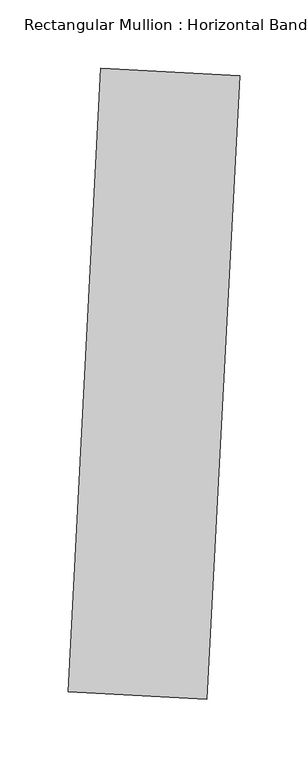
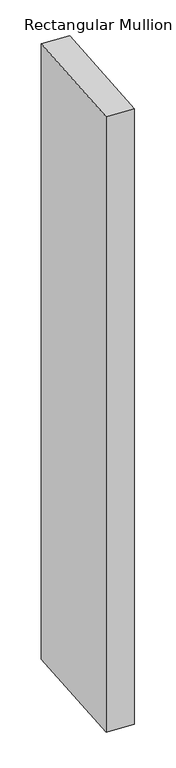
"""IFC4 building model written with IfcOpenShell, lengths in millimetres: member geometry, Rectangular Mullion : Horizontal Band."""

import ifcopenshell
import ifcopenshell.guid

model = None  # the IFC model being written
_history = None  # IfcOwnerHistory: only IFC2X3 demands one
_inside = {}  # id of a spatial element -> (the spatial element, [elements in it])
_under = {}  # id of a project, library or spatial element -> (it, [spatial elements below it])
_declared = {}  # id of a project -> (the project, [libraries it declares])
_typed = {}  # id of a type object -> (the type object, [elements of that type])
_made_of = {}  # id of a material, layer set ... -> (it, [elements and type objects made of it])


def new_model(schema):
    """Start an empty IFC model of exactly this schema.

    Asked for "IFC4X3", IfcOpenShell would pick the latest addendum, in which some entities
    have other attributes; the version numbers below select the first issue.
    IFC2X3 requires an IfcOwnerHistory on every rooted entity: one is made here for all.
    """
    global model, _history
    if schema == "IFC4X3":
        model = ifcopenshell.file(schema_version=(4, 3, 0, 0))
    else:
        model = ifcopenshell.file(schema=schema)
    _inside.clear()
    _under.clear()
    _declared.clear()
    _typed.clear()
    _made_of.clear()
    _history = None
    if model.schema == "IFC2X3":
        org = make("IfcOrganization", Name="unknown")
        user = make(
            "IfcPersonAndOrganization",
            ThePerson=make("IfcPerson", FamilyName="unknown"),
            TheOrganization=org,
        )
        app = make(
            "IfcApplication",
            ApplicationDeveloper=org,
            Version="unknown",
            ApplicationFullName="unknown",
            ApplicationIdentifier="unknown",
        )
        _history = make(
            "IfcOwnerHistory",
            OwningUser=user,
            OwningApplication=app,
            ChangeAction="ADDED",
            CreationDate=0,
        )
    return model


def make(cls, **values):
    """One entity of the class cls with the attributes given. An attribute that is None is left unset."""
    return model.create_entity(
        cls, **{name: value for name, value in values.items() if value is not None}
    )


def rooted(cls, **values):
    """An entity with a GlobalId (a new one), such as an element, a storey or a relation."""
    return make(cls, GlobalId=ifcopenshell.guid.new(), OwnerHistory=_history, **values)


def si_unit(unit_type, name, prefix=None):
    """IfcSIUnit, for example si_unit("LENGTHUNIT", "METRE", prefix="MILLI")."""
    return make("IfcSIUnit", UnitType=unit_type, Prefix=prefix, Name=name)


def assignment(units):
    """IfcUnitAssignment: the units of a project."""
    return None if units is None else make("IfcUnitAssignment", Units=units)


def point(xyz):
    """IfcCartesianPoint."""
    return None if xyz is None else make("IfcCartesianPoint", Coordinates=xyz)


def direction(xyz):
    """IfcDirection."""
    return None if xyz is None else make("IfcDirection", DirectionRatios=xyz)


def frame(location, z_axis=None, x_axis=None):
    """IfcAxis2Placement3D, a coordinate frame: its origin and axes. An axis left out is left unset."""
    return make(
        "IfcAxis2Placement3D",
        Location=point(location),
        Axis=direction(z_axis),
        RefDirection=direction(x_axis),
    )


def origin():
    """The frame at (0, 0, 0) with its axes left unset."""
    return frame((0.0, 0.0, 0.0))


def place(relative_to, where):
    """IfcLocalPlacement: puts the frame where relative to a parent placement (None: the world)."""
    return make(
        "IfcLocalPlacement", PlacementRelTo=relative_to, RelativePlacement=where
    )


def context(
    kind, dimensions, precision=None, world=None, true_north=None, identifier=None
):
    """IfcGeometricRepresentationContext, for example the 3D "Model" context."""
    return make(
        "IfcGeometricRepresentationContext",
        ContextIdentifier=identifier,
        ContextType=kind,
        CoordinateSpaceDimension=dimensions,
        Precision=precision,
        WorldCoordinateSystem=world,
        TrueNorth=true_north,
    )


def project(units=None, contexts=None):
    """IfcProject with its units and contexts."""
    return rooted(
        "IfcProject",
        Name="project",
        RepresentationContexts=contexts,
        UnitsInContext=assignment(units),
    )


def spatial(cls, under=None, at=None, **own):
    """A site, building, storey or space (cls), placed at a placement, below another one or the project."""
    s = rooted(cls, ObjectPlacement=at, **own)
    if under is not None:
        _under.setdefault(under.id(), (under, []))[1].append(s)
    return s


def polyline(points):
    """IfcPolyline through the points."""
    return make("IfcPolyline", Points=[point(p) for p in points])


def outline(outer, holes=None, kind="AREA"):
    """IfcArbitraryClosedProfileDef: a profile drawn as a closed curve; with holes, ...WithVoids."""
    if holes is None:
        return make("IfcArbitraryClosedProfileDef", ProfileType=kind, OuterCurve=outer)
    return make(
        "IfcArbitraryProfileDefWithVoids",
        ProfileType=kind,
        OuterCurve=outer,
        InnerCurves=holes,
    )


def extrude(swept, where, along, depth):
    """IfcExtrudedAreaSolid: the profile swept, set in the frame where, extruded along a direction by depth."""
    return make(
        "IfcExtrudedAreaSolid",
        SweptArea=swept,
        Position=where,
        ExtrudedDirection=direction(along),
        Depth=depth,
    )


def shape(context_of_items, identifier, shape_type, items):
    """IfcShapeRepresentation: the items that make up one representation, for example the "Body"."""
    return make(
        "IfcShapeRepresentation",
        ContextOfItems=context_of_items,
        RepresentationIdentifier=identifier,
        RepresentationType=shape_type,
        Items=items,
    )


def source(mapping_origin, context_of_items, identifier, shape_type, items):
    """IfcRepresentationMap: a shape defined once, which mapped items show again and again."""
    return make(
        "IfcRepresentationMap",
        MappingOrigin=mapping_origin,
        MappedRepresentation=shape(context_of_items, identifier, shape_type, items),
    )


def transform(
    local_origin,
    x_axis=None,
    y_axis=None,
    z_axis=None,
    scale=None,
    scale2=None,
    scale3=None,
    uniform=True,
):
    """IfcCartesianTransformationOperator3D, or its non-uniform kind. x_axis, y_axis, z_axis: its Axis1, 2, 3."""
    if uniform:
        return make(
            "IfcCartesianTransformationOperator3D",
            Axis1=direction(x_axis),
            Axis2=direction(y_axis),
            LocalOrigin=point(local_origin),
            Scale=scale,
            Axis3=direction(z_axis),
        )
    return make(
        "IfcCartesianTransformationOperator3DnonUniform",
        Axis1=direction(x_axis),
        Axis2=direction(y_axis),
        LocalOrigin=point(local_origin),
        Scale=scale,
        Axis3=direction(z_axis),
        Scale2=scale2,
        Scale3=scale3,
    )


def mapped(mapping_source, mapping_target):
    """IfcMappedItem: shows the shape of a source again, moved by a transform."""
    return make(
        "IfcMappedItem", MappingSource=mapping_source, MappingTarget=mapping_target
    )


def made_of(thing, what):
    """Note that an element or type object is made of a material, layer set ...; save() writes the relation."""
    if what is not None:
        _made_of.setdefault(what.id(), (what, []))[1].append(thing)
    return thing


def element(
    cls,
    number,
    at=None,
    inside=None,
    cuts=None,
    type_object=None,
    material=None,
    context=None,
    identifier="Body",
    shape_type=None,
    held_by="IfcProductDefinitionShape",
    body=None,
    shapes=None,
    **own,
):
    """One element of the class cls, such as IfcWall. Its Tag is "e" and its number.

    at: its placement. inside: the storey or other place that contains it. cuts: it is an
    opening in that element (IfcRelVoidsElement). A single representation is given by context,
    identifier, shape_type and body (its items); several are given by shapes. held_by: the class
    of the entity that holds the representations. save() writes the other relations.
    """
    e = rooted(cls, Tag="e%d" % number, ObjectPlacement=at, **own)
    if body is not None:
        shapes = [shape(context, identifier, shape_type, body)]
    if shapes is not None:
        e.Representation = make(held_by, Representations=shapes)
    if inside is not None:
        _inside.setdefault(inside.id(), (inside, []))[1].append(e)
    if cuts is not None:
        rooted(
            "IfcRelVoidsElement", RelatingBuildingElement=cuts, RelatedOpeningElement=e
        )
    if type_object is not None:
        _typed.setdefault(type_object.id(), (type_object, []))[1].append(e)
    return made_of(e, material)


def aggregate(whole, parts):
    """IfcRelAggregates: a whole, such as a stair, and the parts it consists of."""
    return rooted("IfcRelAggregates", RelatingObject=whole, RelatedObjects=parts)


def save(model, path):
    """Write the relations noted so far, then the file.

    IfcRelAggregates (storeys below a building ...), IfcRelContainedInSpatialStructure (elements
    in a storey), IfcRelDefinesByType, IfcRelAssociatesMaterial and IfcRelDeclares: one each for
    every whole, place, type object, material and project.
    """
    for whole, parts in _under.values():
        aggregate(whole, parts)
    for where, things in _inside.values():
        rooted(
            "IfcRelContainedInSpatialStructure",
            RelatedElements=things,
            RelatingStructure=where,
        )
    for kind, things in _typed.values():
        rooted("IfcRelDefinesByType", RelatedObjects=things, RelatingType=kind)
    for what, things in _made_of.values():
        rooted("IfcRelAssociatesMaterial", RelatedObjects=things, RelatingMaterial=what)
    for by, libraries in _declared.values():
        rooted("IfcRelDeclares", RelatingContext=by, RelatedDefinitions=libraries)
    model.write(path)


def rectangular_mullion_horizontal_band_5c9be954(model_context):
    return source(origin(), model_context, "Body", "SweptSolid", [
        extrude(outline(polyline([(62.69438, 301.8280451), (38.7663808, -154.7453782), (-62.69438, -149.4280451), (-38.7663808, 307.1453782), (62.69438, 301.8280451)])), frame((0.0, 0.0, -2412.0054926), z_axis=(0.0, 0.0, 1.0), x_axis=(1.0, 0.0, 0.0)), (0.0, 0.0, 1.0), 2412.0054926),
    ])


if __name__ == "__main__":
    model = new_model("IFC4")
    model_context = context("Model", 3, world=origin())
    ifc_project = project(units=[si_unit("LENGTHUNIT", "METRE", prefix="MILLI")], contexts=[model_context])
    site = spatial("IfcSite", under=ifc_project)
    building = spatial("IfcBuilding", under=site)
    placement = place(None, origin())
    rectangular_mullion_horizontal_band_shape = rectangular_mullion_horizontal_band_5c9be954(model_context)
    element("IfcMember", 1, ObjectType="Rectangular Mullion : Horizontal Band", at=placement, inside=building, context=model_context, shape_type="MappedRepresentation", body=[
        mapped(rectangular_mullion_horizontal_band_shape, transform((0.0, 0.0, 0.0), x_axis=(1.0, 0.0, 0.0), y_axis=(0.0, 1.0, 0.0), z_axis=(0.0, 0.0, 1.0))),
    ])
    save(model, "model.ifc")

# Revit data of these elements
# Type "Rectangular Mullion : Horizontal Band"
#   built-in parameter 1007351 = 0.25 (stored number, unit not read)
#   built-in parameter 1007304 = 1.5 (stored number, unit not read)
#   built-in parameter 1007301 = 0.166667 (stored number, unit not read)
#   built-in parameter 1007300 = 0.166667 (stored number, unit not read)
# Element 1 (IfcMember, "Rectangular Mullion : Horizontal Band")
#   Materials on its faces: "Aluminum"
# Materials
#   "Aluminum": class "Metal", colour RGB 247 247 247, transparency 0, Description = "Aluminum 6061", Cost = 0
